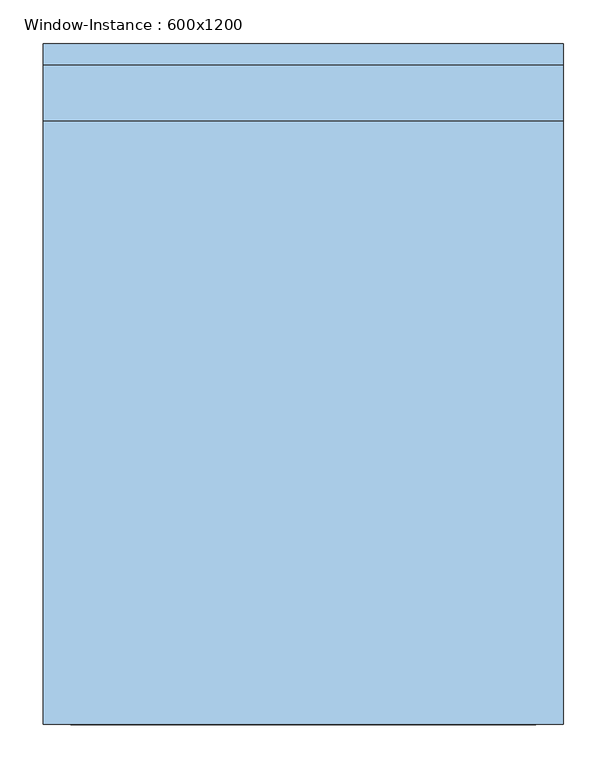
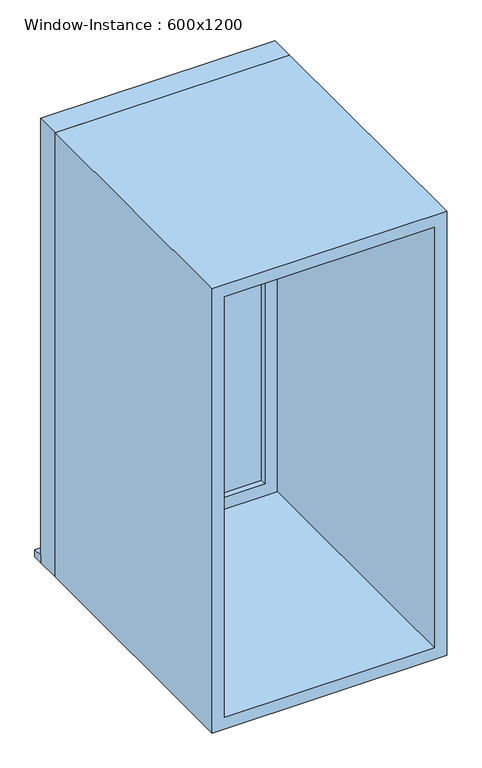
"""IFC4 building model written with IfcOpenShell, lengths in millimetres: window geometry, Window-Instance : 600x1200."""

from ifc_helpers import new_model, si_unit, frame, origin, place, context, project, spatial, polyline, outline, extrude, source, transform, mapped, element, save


def window_instance_600x1200_87f22c1f(model_context):
    return source(origin(), model_context, "Body", "SweptSolid", [
        extrude(outline(polyline([(-338.1, 405.4), (261.9, 405.4), (261.9, 380.0), (-338.1, 380.0), (-338.1, 405.4)])), frame((0.0, 0.0, 900.0), z_axis=(0.0, 0.0, 1.0), x_axis=(1.0, 0.0, 0.0)), (0.0, 0.0, 1.0), 19.05),
        extrude(outline(polyline([(198.4, 331.425), (-274.6, 331.425), (-274.6, 344.125), (198.4, 344.125), (198.4, 331.425)])), frame((0.0, 0.0, 963.5), z_axis=(0.0, 0.0, 1.0), x_axis=(1.0, 0.0, 0.0)), (0.0, 0.0, 1.0), 1073.0),
        extrude(outline(polyline([(2080.95, -319.05), (919.05, -319.05), (919.05, 242.85), (2080.95, 242.85), (2080.95, -319.05)]), holes=[polyline([(2036.5, -274.6), (2036.5, 198.4), (963.5, 198.4), (963.5, -274.6), (2036.5, -274.6)])]), frame((0.0, 315.55, 0.0), z_axis=(0.0, 1.0, 0.0), x_axis=(0.0, 0.0, 1.0)), (0.0, 0.0, 1.0), 44.45),
        extrude(outline(polyline([(2100.0, -338.1), (900.0, -338.1), (900.0, 261.9), (2100.0, 261.9), (2100.0, -338.1)]), holes=[polyline([(2068.25, -306.35), (2068.25, 230.15), (931.75, 230.15), (931.75, -306.35), (2068.25, -306.35)])]), frame((0.0, -380.0, 0.0), z_axis=(0.0, 1.0, 0.0), x_axis=(0.0, 0.0, 1.0)), (0.0, 0.0, 1.0), 695.55),
        extrude(outline(polyline([(2100.0, 261.9), (2100.0, -338.1), (900.0, -338.1), (900.0, 261.9), (2100.0, 261.9)]), holes=[polyline([(2080.95, 242.85), (919.05, 242.85), (919.05, -319.05), (2080.95, -319.05), (2080.95, 242.85)])]), frame((0.0, 315.55, 0.0), z_axis=(0.0, 1.0, 0.0), x_axis=(0.0, 0.0, 1.0)), (0.0, 0.0, 1.0), 64.45),
    ])


if __name__ == "__main__":
    model = new_model("IFC4")
    model_context = context("Model", 3, world=origin())
    ifc_project = project(units=[si_unit("LENGTHUNIT", "METRE", prefix="MILLI")], contexts=[model_context])
    site = spatial("IfcSite", under=ifc_project)
    building = spatial("IfcBuilding", under=site)
    placement = place(None, origin())
    window_instance_600x1200_shape = window_instance_600x1200_87f22c1f(model_context)
    element("IfcWindow", 1, ObjectType="Window-Instance : 600x1200", at=placement, inside=building, context=model_context, shape_type="MappedRepresentation", body=[
        mapped(window_instance_600x1200_shape, transform((0.0, 0.0, 0.0), x_axis=(1.0, 0.0, 0.0), y_axis=(0.0, 1.0, 0.0), z_axis=(0.0, 0.0, 1.0))),
    ])
    save(model, "model.ifc")

# Revit data of these elements
# Type "Window-Instance : 600x1200"
#   Type Mark = "7"
#   Construction Type Id = "GSP4R"
#   Assembly Code = "B2020100"
#   Analytic Construction = "1/8 in Pilkington single glazing"
#   Visual Light Transmittance = 0.9
#   Thermal Resistance (R) = 0.149095 (m²·K)/W
#   Solar Heat Gain Coefficient = 0.86
#   Heat Transfer Coefficient (U) = 6.70716 W/(m²·K)
#   Height [instance default] = 1200 mm
#   Default Sill Height = 900 mm
#   Width [instance default] = 600 mm
#   Window Inset = 20 mm
#   Glass Pane Material = WW-EC-GL-Storefront
#   Sash Material = WW-EC-RGB-White
#   Wall Closure = (empty or 0)
# Element 1 (IfcWindow, "Window-Instance : 600x1200")
#   Materials on its faces: "WW-EC-RGB-White", "WW-EC-GL-Storefront"
# Materials
#   "WW-EC-GL-Storefront": class "Glass", colour RGB 236 240 239, transparency 0.85, Description = "Storefront Glass", Cost = 0
#   "WW-EC-RGB-White": class "Generic", colour RGB 255 255 255, transparency 0, Comments = "If region requests off-white, swith asset color to RGB 231-228-220", Description = "Generic Color", Cost = 0
